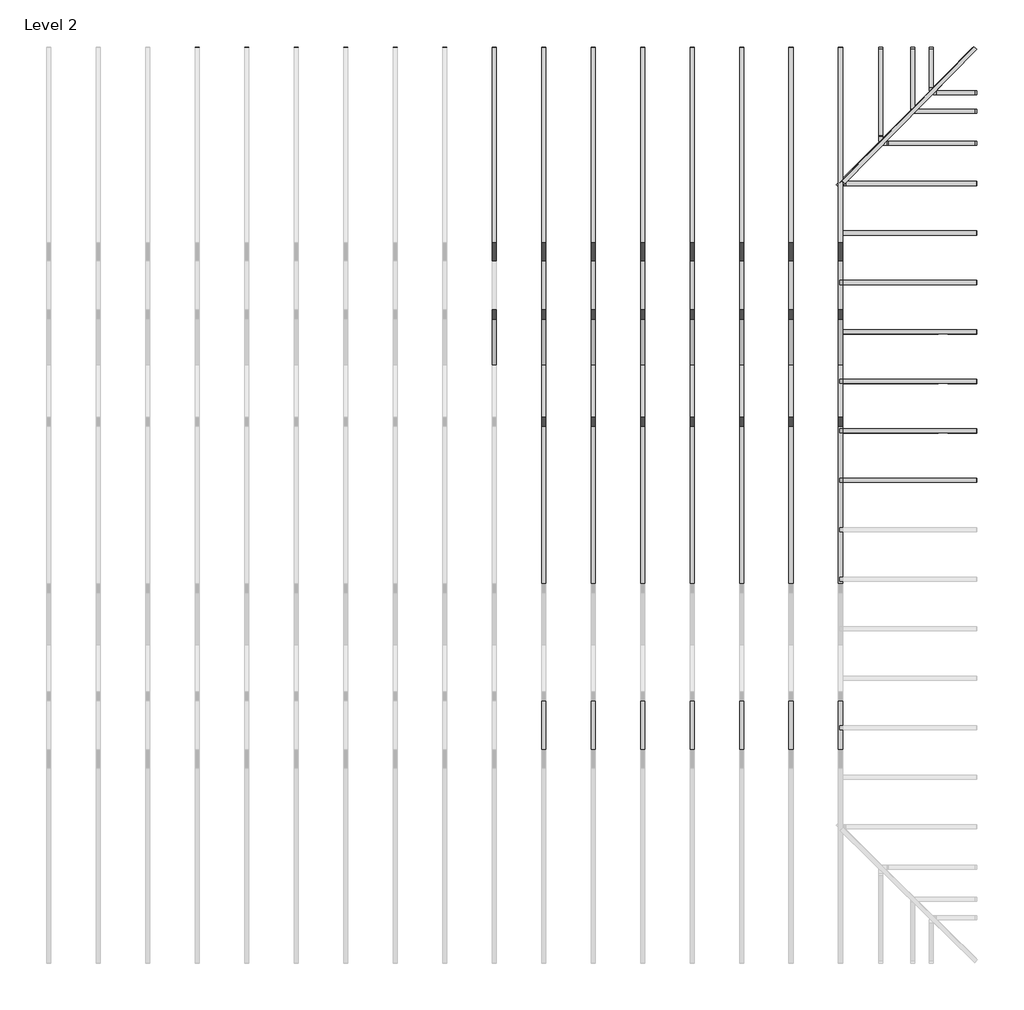
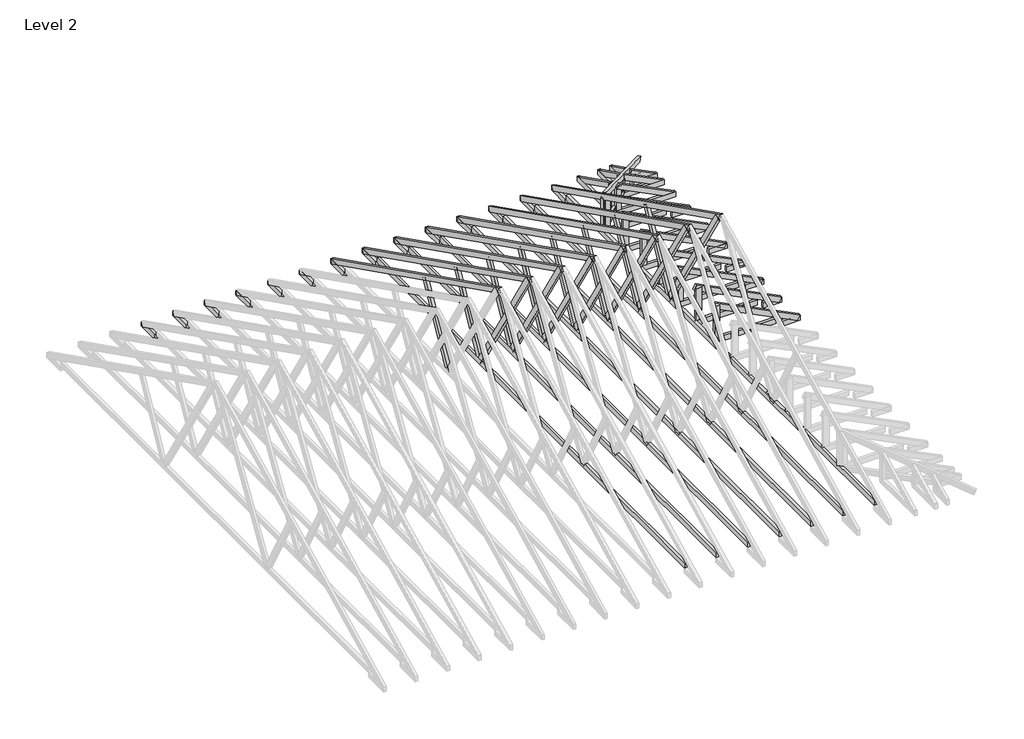
# One storey, part 5 of 5: 93 beams.
"""IFC4 building model written with IfcOpenShell, lengths in millimetres."""

import ifcopenshell
import ifcopenshell.guid

model = None  # the IFC model being written
_history = None  # IfcOwnerHistory: only IFC2X3 demands one
_inside = {}  # id of a spatial element -> (the spatial element, [elements in it])
_under = {}  # id of a project, library or spatial element -> (it, [spatial elements below it])
_declared = {}  # id of a project -> (the project, [libraries it declares])
_typed = {}  # id of a type object -> (the type object, [elements of that type])
_made_of = {}  # id of a material, layer set ... -> (it, [elements and type objects made of it])


def new_model(schema):
    """Start an empty IFC model of exactly this schema.

    Asked for "IFC4X3", IfcOpenShell would pick the latest addendum, in which some entities
    have other attributes; the version numbers below select the first issue.
    IFC2X3 requires an IfcOwnerHistory on every rooted entity: one is made here for all.
    """
    global model, _history
    if schema == "IFC4X3":
        model = ifcopenshell.file(schema_version=(4, 3, 0, 0))
    else:
        model = ifcopenshell.file(schema=schema)
    _inside.clear()
    _under.clear()
    _declared.clear()
    _typed.clear()
    _made_of.clear()
    _history = None
    if model.schema == "IFC2X3":
        org = make("IfcOrganization", Name="unknown")
        user = make(
            "IfcPersonAndOrganization",
            ThePerson=make("IfcPerson", FamilyName="unknown"),
            TheOrganization=org,
        )
        app = make(
            "IfcApplication",
            ApplicationDeveloper=org,
            Version="unknown",
            ApplicationFullName="unknown",
            ApplicationIdentifier="unknown",
        )
        _history = make(
            "IfcOwnerHistory",
            OwningUser=user,
            OwningApplication=app,
            ChangeAction="ADDED",
            CreationDate=0,
        )
    return model


def make(cls, **values):
    """One entity of the class cls with the attributes given. An attribute that is None is left unset."""
    return model.create_entity(
        cls, **{name: value for name, value in values.items() if value is not None}
    )


def rooted(cls, **values):
    """An entity with a GlobalId (a new one), such as an element, a storey or a relation."""
    return make(cls, GlobalId=ifcopenshell.guid.new(), OwnerHistory=_history, **values)


def si_unit(unit_type, name, prefix=None):
    """IfcSIUnit, for example si_unit("LENGTHUNIT", "METRE", prefix="MILLI")."""
    return make("IfcSIUnit", UnitType=unit_type, Prefix=prefix, Name=name)


def assignment(units):
    """IfcUnitAssignment: the units of a project."""
    return None if units is None else make("IfcUnitAssignment", Units=units)


def point(xyz):
    """IfcCartesianPoint."""
    return None if xyz is None else make("IfcCartesianPoint", Coordinates=xyz)


def direction(xyz):
    """IfcDirection."""
    return None if xyz is None else make("IfcDirection", DirectionRatios=xyz)


def frame(location, z_axis=None, x_axis=None):
    """IfcAxis2Placement3D, a coordinate frame: its origin and axes. An axis left out is left unset."""
    return make(
        "IfcAxis2Placement3D",
        Location=point(location),
        Axis=direction(z_axis),
        RefDirection=direction(x_axis),
    )


def origin():
    """The frame at (0, 0, 0) with its axes left unset."""
    return frame((0.0, 0.0, 0.0))


def place(relative_to, where):
    """IfcLocalPlacement: puts the frame where relative to a parent placement (None: the world)."""
    return make(
        "IfcLocalPlacement", PlacementRelTo=relative_to, RelativePlacement=where
    )


def context(
    kind, dimensions, precision=None, world=None, true_north=None, identifier=None
):
    """IfcGeometricRepresentationContext, for example the 3D "Model" context."""
    return make(
        "IfcGeometricRepresentationContext",
        ContextIdentifier=identifier,
        ContextType=kind,
        CoordinateSpaceDimension=dimensions,
        Precision=precision,
        WorldCoordinateSystem=world,
        TrueNorth=true_north,
    )


def project(units=None, contexts=None):
    """IfcProject with its units and contexts."""
    return rooted(
        "IfcProject",
        Name="project",
        RepresentationContexts=contexts,
        UnitsInContext=assignment(units),
    )


def spatial(cls, under=None, at=None, **own):
    """A site, building, storey or space (cls), placed at a placement, below another one or the project."""
    s = rooted(cls, ObjectPlacement=at, **own)
    if under is not None:
        _under.setdefault(under.id(), (under, []))[1].append(s)
    return s


def polyline(points):
    """IfcPolyline through the points."""
    return make("IfcPolyline", Points=[point(p) for p in points])


def outline(outer, holes=None, kind="AREA"):
    """IfcArbitraryClosedProfileDef: a profile drawn as a closed curve; with holes, ...WithVoids."""
    if holes is None:
        return make("IfcArbitraryClosedProfileDef", ProfileType=kind, OuterCurve=outer)
    return make(
        "IfcArbitraryProfileDefWithVoids",
        ProfileType=kind,
        OuterCurve=outer,
        InnerCurves=holes,
    )


def extrude(swept, where, along, depth):
    """IfcExtrudedAreaSolid: the profile swept, set in the frame where, extruded along a direction by depth."""
    return make(
        "IfcExtrudedAreaSolid",
        SweptArea=swept,
        Position=where,
        ExtrudedDirection=direction(along),
        Depth=depth,
    )


def shape(context_of_items, identifier, shape_type, items):
    """IfcShapeRepresentation: the items that make up one representation, for example the "Body"."""
    return make(
        "IfcShapeRepresentation",
        ContextOfItems=context_of_items,
        RepresentationIdentifier=identifier,
        RepresentationType=shape_type,
        Items=items,
    )


def source(mapping_origin, context_of_items, identifier, shape_type, items):
    """IfcRepresentationMap: a shape defined once, which mapped items show again and again."""
    return make(
        "IfcRepresentationMap",
        MappingOrigin=mapping_origin,
        MappedRepresentation=shape(context_of_items, identifier, shape_type, items),
    )


def transform(
    local_origin,
    x_axis=None,
    y_axis=None,
    z_axis=None,
    scale=None,
    scale2=None,
    scale3=None,
    uniform=True,
):
    """IfcCartesianTransformationOperator3D, or its non-uniform kind. x_axis, y_axis, z_axis: its Axis1, 2, 3."""
    if uniform:
        return make(
            "IfcCartesianTransformationOperator3D",
            Axis1=direction(x_axis),
            Axis2=direction(y_axis),
            LocalOrigin=point(local_origin),
            Scale=scale,
            Axis3=direction(z_axis),
        )
    return make(
        "IfcCartesianTransformationOperator3DnonUniform",
        Axis1=direction(x_axis),
        Axis2=direction(y_axis),
        LocalOrigin=point(local_origin),
        Scale=scale,
        Axis3=direction(z_axis),
        Scale2=scale2,
        Scale3=scale3,
    )


def mapped(mapping_source, mapping_target):
    """IfcMappedItem: shows the shape of a source again, moved by a transform."""
    return make(
        "IfcMappedItem", MappingSource=mapping_source, MappingTarget=mapping_target
    )


def made_of(thing, what):
    """Note that an element or type object is made of a material, layer set ...; save() writes the relation."""
    if what is not None:
        _made_of.setdefault(what.id(), (what, []))[1].append(thing)
    return thing


def element(
    cls,
    number,
    at=None,
    inside=None,
    cuts=None,
    type_object=None,
    material=None,
    context=None,
    identifier="Body",
    shape_type=None,
    held_by="IfcProductDefinitionShape",
    body=None,
    shapes=None,
    **own,
):
    """One element of the class cls, such as IfcWall. Its Tag is "e" and its number.

    at: its placement. inside: the storey or other place that contains it. cuts: it is an
    opening in that element (IfcRelVoidsElement). A single representation is given by context,
    identifier, shape_type and body (its items); several are given by shapes. held_by: the class
    of the entity that holds the representations. save() writes the other relations.
    """
    e = rooted(cls, Tag="e%d" % number, ObjectPlacement=at, **own)
    if body is not None:
        shapes = [shape(context, identifier, shape_type, body)]
    if shapes is not None:
        e.Representation = make(held_by, Representations=shapes)
    if inside is not None:
        _inside.setdefault(inside.id(), (inside, []))[1].append(e)
    if cuts is not None:
        rooted(
            "IfcRelVoidsElement", RelatingBuildingElement=cuts, RelatedOpeningElement=e
        )
    if type_object is not None:
        _typed.setdefault(type_object.id(), (type_object, []))[1].append(e)
    return made_of(e, material)


def aggregate(whole, parts):
    """IfcRelAggregates: a whole, such as a stair, and the parts it consists of."""
    return rooted("IfcRelAggregates", RelatingObject=whole, RelatedObjects=parts)


def save(model, path):
    """Write the relations noted so far, then the file.

    IfcRelAggregates (storeys below a building ...), IfcRelContainedInSpatialStructure (elements
    in a storey), IfcRelDefinesByType, IfcRelAssociatesMaterial and IfcRelDeclares: one each for
    every whole, place, type object, material and project.
    """
    for whole, parts in _under.values():
        aggregate(whole, parts)
    for where, things in _inside.values():
        rooted(
            "IfcRelContainedInSpatialStructure",
            RelatedElements=things,
            RelatingStructure=where,
        )
    for kind, things in _typed.values():
        rooted("IfcRelDefinesByType", RelatedObjects=things, RelatingType=kind)
    for what, things in _made_of.values():
        rooted("IfcRelAssociatesMaterial", RelatedObjects=things, RelatingMaterial=what)
    for by, libraries in _declared.values():
        rooted("IfcRelDeclares", RelatingContext=by, RelatedDefinitions=libraries)
    model.write(path)


def beam_b78a0881(model_context):
    return source(origin(), model_context, "Body", "SweptSolid", [
        extrude(outline(polyline([(228.6, 25.4), (228.6, -25.4), (-228.6, -25.4), (-228.6, 25.4), (228.6, 25.4)])), frame((0.0, 0.0, -50.8), z_axis=(0.0, 0.0, 1.0), x_axis=(1.0, 0.0, 0.0)), (0.0, 0.0, 1.0), 101.6),
    ])


def beam_85682148(model_context):
    return source(origin(), model_context, "Body", "SweptSolid", [
        extrude(outline(polyline([(595.8662636, -25.4), (-609.6, -25.4), (-609.6, 25.4), (595.8662636, 25.4), (595.8662636, -25.4)])), frame((0.0, 0.0, -50.8), z_axis=(0.0, 0.0, 1.0), x_axis=(1.0, 0.0, 0.0)), (0.0, 0.0, 1.0), 101.6),
    ])


def beam_f00f3f92(model_context):
    return source(origin(), model_context, "Body", "SweptSolid", [
        extrude(outline(polyline([(393.7, -25.4), (-393.7, -25.4), (-393.7, 25.4), (393.7, 25.4), (393.7, -25.4)])), frame((0.0, 0.0, -50.8), z_axis=(0.0, 0.0, 1.0), x_axis=(1.0, 0.0, 0.0)), (0.0, 0.0, 1.0), 101.6),
    ])


def beam_c3ddfe20(model_context):
    return source(origin(), model_context, "Body", "SweptSolid", [
        extrude(outline(polyline([(393.7, 25.4), (393.7, -25.4), (-368.3, -25.4), (-368.3, 25.4), (393.7, 25.4)])), frame((0.0, 0.0, -50.8), z_axis=(0.0, 0.0, 1.0), x_axis=(1.0, 0.0, 0.0)), (0.0, 0.0, 1.0), 101.6),
    ])


def beam_3de093d9(model_context):
    return source(origin(), model_context, "Body", "SweptSolid", [
        extrude(outline(polyline([(233.4866591, -25.4), (-1464.867127, -25.4), (-1464.867127, 25.4), (233.4866591, 25.4), (233.4866591, -25.4)])), frame((0.0, 0.0, -50.8), z_axis=(0.0, 0.0, 1.0), x_axis=(1.0, 0.0, 0.0)), (0.0, 0.0, 1.0), 101.6),
    ])


def beam_90eea034(model_context):
    return source(origin(), model_context, "Body", "SweptSolid", [
        extrude(outline(polyline([(821.193698, 25.4), (821.193698, -25.4), (-819.5010489, -25.4), (-819.5010489, 25.4), (821.193698, 25.4)])), frame((0.0, 0.0, -50.8), z_axis=(0.0, 0.0, 1.0), x_axis=(1.0, 0.0, 0.0)), (0.0, 0.0, 1.0), 101.6),
    ])


def beam_a4242642(model_context):
    return source(origin(), model_context, "Body", "SweptSolid", [
        extrude(outline(polyline([(5145.3336481, 25.4), (5145.3336481, -25.4), (-5145.3336481, -25.4), (-5145.3336481, 25.4), (5145.3336481, 25.4)])), frame((0.0, 0.0, -50.8), z_axis=(0.0, 0.0, 1.0), x_axis=(1.0, 0.0, 0.0)), (0.0, 0.0, 1.0), 101.6),
    ])


def beam_fc8bf4ae(model_context):
    return source(origin(), model_context, "Body", "SweptSolid", [
        extrude(outline(polyline([(1562.6646551, 25.4), (1562.6646551, -25.4), (-1550.1468127, -25.4), (-1550.1468127, 25.4), (1562.6646551, 25.4)])), frame((0.0, 0.0, -50.8), z_axis=(0.0, 0.0, 1.0), x_axis=(1.0, 0.0, 0.0)), (0.0, 0.0, 1.0), 101.6),
    ])


def beam_87710fdd(model_context):
    return source(origin(), model_context, "Body", "SweptSolid", [
        extrude(outline(polyline([(147.1272806, 25.4), (147.1272806, -25.4), (-142.875, -25.4), (-142.875, 25.4), (147.1272806, 25.4)])), frame((0.0, 0.0, -50.8), z_axis=(0.0, 0.0, 1.0), x_axis=(1.0, 0.0, 0.0)), (0.0, 0.0, 1.0), 101.6),
    ])


def beam_7b8fa6d1(model_context):
    return source(origin(), model_context, "Body", "SweptSolid", [
        extrude(outline(polyline([(270.7395597, 25.4), (270.7395597, -25.4), (-219.9395597, -25.4), (-219.9395597, 25.4), (270.7395597, 25.4)])), frame((0.0, 0.0, -50.8), z_axis=(0.0, 0.0, 1.0), x_axis=(1.0, 0.0, 0.0)), (0.0, 0.0, 1.0), 101.6),
    ])


def beam_42a29ae5(model_context):
    return source(origin(), model_context, "Body", "SweptSolid", [
        extrude(outline(polyline([(270.7395597, -25.4), (-219.9395597, -25.4), (-219.9395597, 25.4), (270.7395597, 25.4), (270.7395597, -25.4)])), frame((0.0, 0.0, -50.8), z_axis=(0.0, 0.0, 1.0), x_axis=(1.0, 0.0, 0.0)), (0.0, 0.0, 1.0), 101.6),
    ])


def beam_11c5b8ca(model_context):
    return source(origin(), model_context, "Body", "SweptSolid", [
        extrude(outline(polyline([(147.1272806, -25.4), (-142.875, -25.4), (-142.875, 25.4), (147.1272806, 25.4), (147.1272806, -25.4)])), frame((0.0, 0.0, -50.8), z_axis=(0.0, 0.0, 1.0), x_axis=(1.0, 0.0, 0.0)), (0.0, 0.0, 1.0), 101.6),
    ])


def beam_a8bd1fc0(model_context):
    return source(origin(), model_context, "Body", "SweptSolid", [
        extrude(outline(polyline([(571.5, -25.4), (-609.6, -25.4), (-609.6, 25.4), (571.5, 25.4), (571.5, -25.4)])), frame((0.0, 0.0, -50.8), z_axis=(0.0, 0.0, 1.0), x_axis=(1.0, 0.0, 0.0)), (0.0, 0.0, 1.0), 101.6),
    ])


def beam_f5027b49(model_context):
    return source(origin(), model_context, "Body", "SweptSolid", [
        extrude(outline(polyline([(571.5, 25.4), (571.5, -25.4), (-584.2, -25.4), (-584.2, 25.4), (571.5, 25.4)])), frame((0.0, 0.0, -50.8), z_axis=(0.0, 0.0, 1.0), x_axis=(1.0, 0.0, 0.0)), (0.0, 0.0, 1.0), 101.6),
    ])


def beam_78ff79ac(model_context):
    return source(origin(), model_context, "Body", "SweptSolid", [
        extrude(outline(polyline([(365.3019367, -25.4), (-314.5019367, -25.4), (-314.5019367, 25.4), (365.3019367, 25.4), (365.3019367, -25.4)])), frame((0.0, 0.0, -50.8), z_axis=(0.0, 0.0, 1.0), x_axis=(1.0, 0.0, 0.0)), (0.0, 0.0, 1.0), 101.6),
    ])


def beam_99e5442a(model_context):
    return source(origin(), model_context, "Body", "SweptSolid", [
        extrude(outline(polyline([(350.5042173, -25.4), (-295.4519367, -25.4), (-295.4519367, 25.4), (350.5042173, 25.4), (350.5042173, -25.4)])), frame((0.0, 0.0, -50.8), z_axis=(0.0, 0.0, 1.0), x_axis=(1.0, 0.0, 0.0)), (0.0, 0.0, 1.0), 101.6),
    ])


def beam_38e3f9e5(model_context):
    return source(origin(), model_context, "Body", "SweptSolid", [
        extrude(outline(polyline([(595.8662636, -25.4), (-548.2789755, -25.4), (-548.2789755, 25.4), (595.8662636, 25.4), (595.8662636, -25.4)])), frame((0.0, 0.0, -50.8), z_axis=(0.0, 0.0, 1.0), x_axis=(1.0, 0.0, 0.0)), (0.0, 0.0, 1.0), 101.6),
    ])


def beam_7aad778a(model_context):
    return source(origin(), model_context, "Body", "SweptSolid", [
        extrude(outline(polyline([(307.975, -25.4), (-47.625, -25.4), (-47.625, 25.4), (307.975, 25.4), (307.975, -25.4)])), frame((0.0, 0.0, -50.8), z_axis=(0.0, 0.0, 1.0), x_axis=(1.0, 0.0, 0.0)), (0.0, 0.0, 1.0), 101.6),
    ])


def beam_878446a4(model_context):
    return source(origin(), model_context, "Body", "SweptSolid", [
        extrude(outline(polyline([(63.8057136, 25.4), (63.8057136, -25.4), (-59.553433, -25.4), (-59.553433, 25.4), (63.8057136, 25.4)])), frame((0.0, 0.0, -50.8), z_axis=(0.0, 0.0, 1.0), x_axis=(1.0, 0.0, 0.0)), (0.0, 0.0, 1.0), 101.6),
    ])


def beam_bc99fd75(model_context):
    return source(origin(), model_context, "Body", "SweptSolid", [
        extrude(outline(polyline([(222.3387319, 25.4), (222.3387319, -25.4), (-231.775, -25.4), (-231.775, 25.4), (222.3387319, 25.4)])), frame((0.0, 0.0, -50.8), z_axis=(0.0, 0.0, 1.0), x_axis=(1.0, 0.0, 0.0)), (0.0, 0.0, 1.0), 101.6),
    ])


def beam_efe25585(model_context):
    return source(origin(), model_context, "Body", "SweptSolid", [
        extrude(outline(polyline([(222.3387319, -25.4), (-231.775, -25.4), (-231.775, 25.4), (222.3387319, 25.4), (222.3387319, -25.4)])), frame((0.0, 0.0, -50.8), z_axis=(0.0, 0.0, 1.0), x_axis=(1.0, 0.0, 0.0)), (0.0, 0.0, 1.0), 101.6),
    ])


def beam_dfed05dc(model_context):
    return source(origin(), model_context, "Body", "SweptSolid", [
        extrude(outline(polyline([(63.8057136, -25.4), (-59.553433, -25.4), (-59.553433, 25.4), (63.8057136, 25.4), (63.8057136, -25.4)])), frame((0.0, 0.0, -50.8), z_axis=(0.0, 0.0, 1.0), x_axis=(1.0, 0.0, 0.0)), (0.0, 0.0, 1.0), 101.6),
    ])


model = new_model("IFC4")

# Units and contexts
model_context = context("Model", 3, world=origin())
ifc_project = project(units=[si_unit("LENGTHUNIT", "METRE", prefix="MILLI")], contexts=[model_context])

# Site, building, storey
site = spatial("IfcSite", under=ifc_project)
building = spatial("IfcBuilding", under=site)
storey = spatial("IfcBuildingStorey", under=building, Name="Level 2", Elevation=2768.6)

# Beams
placement = place(None, origin())
element("IfcBeam", 1, ObjectType="Dimension Lumber : BLDG 6241 2X4\" TRUSS MEMBER", at=placement, inside=storey, context=model_context, shape_type="SweptSolid", body=[
    extrude(outline(polyline([(0.0, -50.8), (0.0, 0.0), (6302.2496334, 0.0), (6302.2496334, -50.8), (0.0, -50.8)])), frame((-3805.814829, -17.2791662, 5496.1115355), z_axis=(0.0, 0.4472135954999557, 0.894427190999917), x_axis=(0.0, 0.894427190999917, -0.4472135954999557)), (0.0, 0.0, 1.0), 101.6),
])
element("IfcBeam", 2, ObjectType="Dimension Lumber : BLDG 6241 2X4\" TRUSS MEMBER", at=placement, inside=storey, context=model_context, shape_type="SweptSolid", body=[
    extrude(outline(polyline([(0.0, -50.8), (0.0, 0.0), (6302.2496334, 0.0), (6302.2496334, -50.8), (0.0, -50.8)])), frame((-3196.214829, -17.2791662, 5496.1115355), z_axis=(0.0, 0.4472135954999561, 0.8944271909999169), x_axis=(0.0, 0.8944271909999169, -0.4472135954999561)), (0.0, 0.0, 1.0), 101.6),
])
element("IfcBeam", 3, ObjectType="Dimension Lumber : BLDG 6241 2X4\" TRUSS MEMBER", at=placement, inside=storey, context=model_context, shape_type="SweptSolid", body=[
    extrude(outline(polyline([(0.0, -50.8), (0.0, 0.0), (6302.2496334, 0.0), (6302.2496334, -50.8), (0.0, -50.8)])), frame((-2586.614829, -17.2791662, 5496.1115355), z_axis=(0.0, 0.44721359549995593, 0.894427190999917), x_axis=(0.0, 0.894427190999917, -0.44721359549995593)), (0.0, 0.0, 1.0), 101.6),
])
element("IfcBeam", 4, ObjectType="Dimension Lumber : BLDG 6241 2X4\" TRUSS MEMBER", at=placement, inside=storey, context=model_context, shape_type="SweptSolid", body=[
    extrude(outline(polyline([(0.0, -50.8), (0.0, 0.0), (6302.2496334, 0.0), (6302.2496334, -50.8), (0.0, -50.8)])), frame((-1977.014829, -17.2791662, 5496.1115355), z_axis=(0.0, 0.447213595499956, 0.8944271909999169), x_axis=(0.0, 0.8944271909999169, -0.447213595499956)), (0.0, 0.0, 1.0), 101.6),
])
element("IfcBeam", 5, ObjectType="Dimension Lumber : BLDG 6241 2X4\" TRUSS MEMBER", at=placement, inside=storey, context=model_context, shape_type="SweptSolid", body=[
    extrude(outline(polyline([(0.0, -50.8), (0.0, 0.0), (6302.2496334, 0.0), (6302.2496334, -50.8), (0.0, -50.8)])), frame((-1367.414829, -17.2791662, 5496.1115355), z_axis=(0.0, 0.44721359549995593, 0.894427190999917), x_axis=(0.0, 0.894427190999917, -0.44721359549995593)), (0.0, 0.0, 1.0), 101.6),
])
element("IfcBeam", 6, ObjectType="Dimension Lumber : BLDG 6241 2X4\" TRUSS MEMBER", at=placement, inside=storey, context=model_context, shape_type="SweptSolid", body=[
    extrude(outline(polyline([(0.0, -50.8), (0.0, 0.0), (6302.2496334, 0.0), (6302.2496334, -50.8), (0.0, -50.8)])), frame((-757.814829, -17.2791662, 5496.1115355), z_axis=(0.0, 0.4472135954999558, 0.894427190999917), x_axis=(0.0, 0.894427190999917, -0.4472135954999558)), (0.0, 0.0, 1.0), 101.6),
])
element("IfcBeam", 7, ObjectType="Dimension Lumber : BLDG 6241 2X4\" TRUSS MEMBER", at=placement, inside=storey, context=model_context, shape_type="SweptSolid", body=[
    extrude(outline(polyline([(0.0, -50.8), (0.0, 0.0), (6302.2496334, 0.0), (6302.2496334, -50.8), (0.0, -50.8)])), frame((-148.214829, -17.2791662, 5496.1115355), z_axis=(0.0, 0.4472135954999557, 0.894427190999917), x_axis=(0.0, 0.894427190999917, -0.4472135954999557)), (0.0, 0.0, 1.0), 101.6),
])
element("IfcBeam", 8, ObjectType="Dimension Lumber : BLDG 6241 2X4\" TRUSS MEMBER", at=placement, inside=storey, context=model_context, shape_type="SweptSolid", body=[
    extrude(outline(polyline([(0.0, -50.8), (0.0, 0.0), (6302.2496334, 0.0), (6302.2496334, -50.8), (0.0, -50.8)])), frame((461.385171, -17.2791662, 5496.1115355), z_axis=(0.0, 0.4472135954999561, 0.8944271909999169), x_axis=(0.0, 0.8944271909999169, -0.4472135954999561)), (0.0, 0.0, 1.0), 101.6),
])
element("IfcBeam", 9, ObjectType="Dimension Lumber : BLDG 6241 2X4\" TRUSS MEMBER", at=placement, inside=storey, context=model_context, shape_type="SweptSolid", body=[
    extrude(outline(polyline([(0.0, 50.8), (1828.8, 50.8), (1828.8, 0.0), (0.0, 0.0), (0.0, 50.8)])), frame((2110.9853106, 3404.3284114, 2681.1076769), z_axis=(0.44721359549995937, 0.0, 0.8944271909999152), x_axis=(-0.8944271909999152, 0.0, 0.44721359549995937)), (0.0, 0.0, 1.0), 101.6),
])
element("IfcBeam", 10, ObjectType="Dimension Lumber : BLDG 6241 2X4\" TRUSS MEMBER", at=placement, inside=storey, context=model_context, shape_type="SweptSolid", body=[
    extrude(outline(polyline([(0.0, 50.8000001), (2461.5286969, 50.8), (2461.528697, 0.0), (0.0, 0.0), (0.0, 50.8000001)])), frame((510.3258967, 3962.9132559, 3515.7397288), z_axis=(0.25320527715849206, 0.22183093198504344, 0.9416358772018716), x_axis=(0.6604274920267093, 0.6716162760239278, -0.33580813801196396)), (0.0, 0.0, 1.0), 101.6),
])
element("IfcBeam", 11, ObjectType="Dimension Lumber : BLDG 6241 2X4\" TRUSS MEMBER", at=placement, inside=storey, context=model_context, shape_type="SweptSolid", body=[
    extrude(outline(polyline([(0.0, 50.8), (1203.6219076, 50.8), (1203.6219076, 0.0), (0.0, 0.0), (0.0, 50.8)])), frame((2112.5153243, 4509.2284114, 2680.3426701), z_axis=(0.44721359549995937, 0.0, 0.8944271909999152), x_axis=(-0.8944271909999152, 0.0, 0.44721359549995937)), (0.0, 0.0, 1.0), 101.6),
])
element("IfcBeam", 12, ObjectType="Dimension Lumber : BLDG 6241 2X4\" TRUSS MEMBER", at=placement, inside=storey, context=model_context, shape_type="SweptSolid", body=[
    extrude(outline(polyline([(0.0, 50.8), (844.55, 50.8), (844.55, 0.0), (0.0, 0.0), (0.0, 50.8)])), frame((2117.2589031, 4902.9284114, 2677.9708807), z_axis=(0.4472135954999599, 0.0, 0.894427190999915), x_axis=(-0.894427190999915, 0.0, 0.4472135954999599)), (0.0, 0.0, 1.0), 101.6),
])
element("IfcBeam", 13, ObjectType="Dimension Lumber : BLDG 6241 2X4\" TRUSS MEMBER", at=placement, inside=storey, context=model_context, shape_type="SweptSolid", body=[
    extrude(outline(polyline([(0.0, 50.8), (1787.5128973, 50.8), (1787.5128973, 0.0), (0.0, 0.0), (0.0, 50.8)])), frame((2110.9853106, 4013.9284114, 2681.1076769), z_axis=(0.44721359549995937, 0.0, 0.8944271909999152), x_axis=(-0.8944271909999152, 0.0, 0.44721359549995937)), (0.0, 0.0, 1.0), 101.6),
])
element("IfcBeam", 14, ObjectType="Dimension Lumber : BLDG 6241 2X4\" TRUSS MEMBER", at=placement, inside=storey, context=model_context, shape_type="SweptSolid", body=[
    extrude(outline(polyline([(0.0, 50.8), (1828.8, 50.8), (1828.8, 0.0), (0.0, 0.0), (0.0, 50.8)])), frame((2110.9853106, 2794.7284114, 2681.1076769), z_axis=(0.44721359549995937, 0.0, 0.8944271909999152), x_axis=(-0.8944271909999152, 0.0, 0.44721359549995937)), (0.0, 0.0, 1.0), 101.6),
])
element("IfcBeam", 15, ObjectType="Dimension Lumber : BLDG 6241 2X4\" TRUSS MEMBER", at=placement, inside=storey, context=model_context, shape_type="SweptSolid", body=[
    extrude(outline(polyline([(0.0, 50.8), (1828.8, 50.8), (1828.8, 0.0), (0.0, 0.0), (0.0, 50.8)])), frame((2110.9853106, 2185.1284114, 2681.1076769), z_axis=(0.44721359549995937, 0.0, 0.8944271909999152), x_axis=(-0.8944271909999152, 0.0, 0.44721359549995937)), (0.0, 0.0, 1.0), 101.6),
])
element("IfcBeam", 16, ObjectType="Dimension Lumber : BLDG 6241 2X4\" TRUSS MEMBER", at=placement, inside=storey, context=model_context, shape_type="SweptSolid", body=[
    extrude(outline(polyline([(0.0, 50.8), (1828.8, 50.8), (1828.8, 0.0), (0.0, 0.0), (0.0, 50.8)])), frame((2110.9853106, 1575.5284114, 2681.1076769), z_axis=(0.44721359549995937, 0.0, 0.8944271909999152), x_axis=(-0.8944271909999152, 0.0, 0.44721359549995937)), (0.0, 0.0, 1.0), 101.6),
])
element("IfcBeam", 17, ObjectType="Dimension Lumber : BLDG 6241 2X4\" TRUSS MEMBER", at=placement, inside=storey, context=model_context, shape_type="SweptSolid", body=[
    extrude(outline(polyline([(0.0, 50.8), (1828.8, 50.8), (1828.8, 0.0), (0.0, 0.0), (0.0, 50.8)])), frame((2110.9853106, 965.9284114, 2681.1076769), z_axis=(0.44721359549995937, 0.0, 0.8944271909999152), x_axis=(-0.8944271909999152, 0.0, 0.44721359549995937)), (0.0, 0.0, 1.0), 101.6),
])
element("IfcBeam", 18, ObjectType="Dimension Lumber : BLDG 6241 2X4\" TRUSS MEMBER", at=placement, inside=storey, context=model_context, shape_type="SweptSolid", body=[
    extrude(outline(polyline([(0.0, 50.8), (1828.8, 50.8), (1828.8, 0.0), (0.0, 0.0), (0.0, 50.8)])), frame((2110.9853106, 356.3284114, 2681.1076769), z_axis=(0.44721359549995937, 0.0, 0.8944271909999152), x_axis=(-0.8944271909999152, 0.0, 0.44721359549995937)), (0.0, 0.0, 1.0), 101.6),
])
element("IfcBeam", 19, ObjectType="Dimension Lumber : BLDG 6241 2X4\" TRUSS MEMBER", at=placement, inside=storey, context=model_context, shape_type="SweptSolid", body=[
    extrude(outline(polyline([(0.0, -50.8), (0.0, 0.0), (1203.6219076, 0.0), (1203.6219076, -50.8), (0.0, -50.8)])), frame((1007.485171, 5614.2585647, 2680.3426701), z_axis=(0.0, 0.44721359549995937, 0.8944271909999152), x_axis=(0.0, -0.8944271909999152, 0.44721359549995937)), (0.0, 0.0, 1.0), 101.6),
])
element("IfcBeam", 20, ObjectType="Dimension Lumber : BLDG 6241 2X4\" TRUSS MEMBER", at=placement, inside=storey, context=model_context, shape_type="SweptSolid", body=[
    extrude(outline(polyline([(0.0, -50.8), (0.0, 0.0), (844.55, 0.0), (844.55, -50.8), (0.0, -50.8)])), frame((1401.185171, 5619.0021435, 2677.9708807), z_axis=(0.0, 0.4472135954999599, 0.894427190999915), x_axis=(0.0, -0.894427190999915, 0.4472135954999599)), (0.0, 0.0, 1.0), 101.6),
])
element("IfcBeam", 21, ObjectType="Dimension Lumber : BLDG 6241 2X4\" TRUSS MEMBER", at=placement, inside=storey, context=model_context, shape_type="SweptSolid", body=[
    extrude(outline(polyline([(0.0, 50.8), (546.1, 50.8), (546.1, 0.0), (0.0, 0.0), (0.0, 50.8)])), frame((2116.9461224, 5131.5284114, 2678.127271), z_axis=(0.4472135954999593, 0.0, 0.8944271909999153), x_axis=(-0.8944271909999153, 0.0, 0.4472135954999593)), (0.0, 0.0, 1.0), 101.6),
])
element("IfcBeam", 22, ObjectType="Dimension Lumber : BLDG 6241 2X4\" TRUSS MEMBER", at=placement, inside=storey, context=model_context, shape_type="SweptSolid", body=[
    extrude(outline(polyline([(0.0, -50.8), (0.0, 0.0), (546.1, 0.0), (546.1, -50.8), (0.0, -50.8)])), frame((1629.785171, 5618.6893628, 2678.127271), z_axis=(0.0, 0.4472135954999592, 0.8944271909999153), x_axis=(0.0, -0.8944271909999153, 0.4472135954999592)), (0.0, 0.0, 1.0), 101.6),
])
beam_shape = beam_b78a0881(model_context)
element("IfcBeam", 23, ObjectType="Dimension Lumber : BLDG 6241 2X4\" TRUSS MEMBER", at=placement, inside=storey, context=model_context, shape_type="MappedRepresentation", body=[
    mapped(beam_shape, transform((-7438.014829, 5436.3284114, 2717.8), x_axis=(0.0, -1.0, 0.0), y_axis=(1.0, 0.0, 0.0), z_axis=(0.0, 0.0, 1.0))),
])
element("IfcBeam", 24, ObjectType="Dimension Lumber : BLDG 6241 2X4\" TRUSS MEMBER", at=placement, inside=storey, context=model_context, shape_type="MappedRepresentation", body=[
    mapped(beam_shape, transform((-6828.414829, 5436.3284114, 2717.8), x_axis=(0.0, -1.0, 0.0), y_axis=(1.0, 0.0, 0.0), z_axis=(0.0, 0.0, 1.0))),
])
element("IfcBeam", 25, ObjectType="Dimension Lumber : BLDG 6241 2X4\" TRUSS MEMBER", at=placement, inside=storey, context=model_context, shape_type="MappedRepresentation", body=[
    mapped(beam_shape, transform((-6218.814829, 5436.3284114, 2717.8), x_axis=(0.0, -1.0, 0.0), y_axis=(1.0, 0.0, 0.0), z_axis=(0.0, 0.0, 1.0))),
])
element("IfcBeam", 26, ObjectType="Dimension Lumber : BLDG 6241 2X4\" TRUSS MEMBER", at=placement, inside=storey, context=model_context, shape_type="MappedRepresentation", body=[
    mapped(beam_shape, transform((-5609.214829, 5436.3284114, 2717.8), x_axis=(0.0, -1.0, 0.0), y_axis=(1.0, 0.0, 0.0), z_axis=(0.0, 0.0, 1.0))),
])
element("IfcBeam", 27, ObjectType="Dimension Lumber : BLDG 6241 2X4\" TRUSS MEMBER", at=placement, inside=storey, context=model_context, shape_type="MappedRepresentation", body=[
    mapped(beam_shape, transform((-4999.614829, 5436.3284114, 2717.8), x_axis=(0.0, -1.0, 0.0), y_axis=(1.0, 0.0, 0.0), z_axis=(0.0, 0.0, 1.0))),
])
element("IfcBeam", 28, ObjectType="Dimension Lumber : BLDG 6241 2X4\" TRUSS MEMBER", at=placement, inside=storey, context=model_context, shape_type="MappedRepresentation", body=[
    mapped(beam_shape, transform((-4390.014829, 5436.3284114, 2717.8), x_axis=(0.0, -1.0, 0.0), y_axis=(1.0, 0.0, 0.0), z_axis=(0.0, 0.0, 1.0))),
])
element("IfcBeam", 29, ObjectType="Dimension Lumber : BLDG 6241 2X4\" TRUSS MEMBER", at=placement, inside=storey, context=model_context, shape_type="MappedRepresentation", body=[
    mapped(beam_shape, transform((-3780.414829, 5436.3284114, 2717.8), x_axis=(0.0, -1.0, 0.0), y_axis=(1.0, 0.0, 0.0), z_axis=(0.0, 0.0, 1.0))),
])
element("IfcBeam", 30, ObjectType="Dimension Lumber : BLDG 6241 2X4\" TRUSS MEMBER", at=placement, inside=storey, context=model_context, shape_type="MappedRepresentation", body=[
    mapped(beam_shape, transform((-3170.814829, 5436.3284114, 2717.8), x_axis=(0.0, -1.0, 0.0), y_axis=(1.0, 0.0, 0.0), z_axis=(0.0, 0.0, 1.0))),
])
element("IfcBeam", 31, ObjectType="Dimension Lumber : BLDG 6241 2X4\" TRUSS MEMBER", at=placement, inside=storey, context=model_context, shape_type="MappedRepresentation", body=[
    mapped(beam_shape, transform((-2561.214829, 5436.3284114, 2717.8), x_axis=(0.0, -1.0, 0.0), y_axis=(1.0, 0.0, 0.0), z_axis=(0.0, 0.0, 1.0))),
])
element("IfcBeam", 32, ObjectType="Dimension Lumber : BLDG 6241 2X4\" TRUSS MEMBER", at=placement, inside=storey, context=model_context, shape_type="MappedRepresentation", body=[
    mapped(beam_shape, transform((-1951.614829, 5436.3284114, 2717.8), x_axis=(0.0, -1.0, 0.0), y_axis=(1.0, 0.0, 0.0), z_axis=(0.0, 0.0, 1.0))),
])
element("IfcBeam", 33, ObjectType="Dimension Lumber : BLDG 6241 2X4\" TRUSS MEMBER", at=placement, inside=storey, context=model_context, shape_type="MappedRepresentation", body=[
    mapped(beam_shape, transform((-1342.014829, 5436.3284114, 2717.8), x_axis=(0.0, -1.0, 0.0), y_axis=(1.0, 0.0, 0.0), z_axis=(0.0, 0.0, 1.0))),
])
element("IfcBeam", 34, ObjectType="Dimension Lumber : BLDG 6241 2X4\" TRUSS MEMBER", at=placement, inside=storey, context=model_context, shape_type="MappedRepresentation", body=[
    mapped(beam_shape, transform((-732.414829, 5436.3284114, 2717.8), x_axis=(0.0, -1.0, 0.0), y_axis=(1.0, 0.0, 0.0), z_axis=(0.0, 0.0, 1.0))),
])
element("IfcBeam", 35, ObjectType="Dimension Lumber : BLDG 6241 2X4\" TRUSS MEMBER", at=placement, inside=storey, context=model_context, shape_type="MappedRepresentation", body=[
    mapped(beam_shape, transform((-122.814829, 5436.3284114, 2717.8), x_axis=(0.0, -1.0, 0.0), y_axis=(1.0, 0.0, 0.0), z_axis=(0.0, 0.0, 1.0))),
])
element("IfcBeam", 36, ObjectType="Dimension Lumber : BLDG 6241 2X4\" TRUSS MEMBER", at=placement, inside=storey, context=model_context, shape_type="MappedRepresentation", body=[
    mapped(beam_shape, transform((486.785171, 5436.3284114, 2717.8), x_axis=(0.0, -1.0, 0.0), y_axis=(1.0, 0.0, 0.0), z_axis=(0.0, 0.0, 1.0))),
])
beam_2_shape = beam_85682148(model_context)
element("IfcBeam", 37, ObjectType="Dimension Lumber : BLDG 6241 2X4\" TRUSS MEMBER", at=placement, inside=storey, context=model_context, shape_type="MappedRepresentation", body=[
    mapped(beam_2_shape, transform((1096.385171, 3378.9284114, 2819.4), x_axis=(1.0, 0.0, 0.0), y_axis=(0.0, 1.0, 0.0), z_axis=(0.0, 0.0, 1.0))),
])
element("IfcBeam", 38, ObjectType="Dimension Lumber : BLDG 6241 2X4\" TRUSS MEMBER", at=placement, inside=storey, context=model_context, shape_type="MappedRepresentation", body=[
    mapped(beam_2_shape, transform((1096.385171, 2769.3284114, 2819.4), x_axis=(1.0, 0.0, 0.0), y_axis=(0.0, 1.0, 0.0), z_axis=(0.0, 0.0, 1.0))),
])
element("IfcBeam", 39, ObjectType="Dimension Lumber : BLDG 6241 2X4\" TRUSS MEMBER", at=placement, inside=storey, context=model_context, shape_type="MappedRepresentation", body=[
    mapped(beam_2_shape, transform((1096.385171, 2159.7284114, 2819.4), x_axis=(1.0, 0.0, 0.0), y_axis=(0.0, 1.0, 0.0), z_axis=(0.0, 0.0, 1.0))),
])
element("IfcBeam", 40, ObjectType="Dimension Lumber : BLDG 6241 2X4\" TRUSS MEMBER", at=placement, inside=storey, context=model_context, shape_type="MappedRepresentation", body=[
    mapped(beam_2_shape, transform((1096.385171, 1550.1284114, 2819.4), x_axis=(1.0, 0.0, 0.0), y_axis=(0.0, 1.0, 0.0), z_axis=(0.0, 0.0, 1.0))),
])
element("IfcBeam", 41, ObjectType="Dimension Lumber : BLDG 6241 2X4\" TRUSS MEMBER", at=placement, inside=storey, context=model_context, shape_type="MappedRepresentation", body=[
    mapped(beam_2_shape, transform((1096.385171, 940.5284114, 2819.4), x_axis=(1.0, 0.0, 0.0), y_axis=(0.0, 1.0, 0.0), z_axis=(0.0, 0.0, 1.0))),
])
element("IfcBeam", 42, ObjectType="Dimension Lumber : BLDG 6241 2X4\" TRUSS MEMBER", at=placement, inside=storey, context=model_context, shape_type="MappedRepresentation", body=[
    mapped(beam_2_shape, transform((1096.385171, 330.9284114, 2819.4), x_axis=(1.0, 0.0, 0.0), y_axis=(0.0, 1.0, 0.0), z_axis=(0.0, 0.0, 1.0))),
])
beam_3_shape = beam_f00f3f92(model_context)
element("IfcBeam", 43, ObjectType="Dimension Lumber : BLDG 6241 2X4\" TRUSS MEMBER", at=placement, inside=storey, context=model_context, shape_type="MappedRepresentation", body=[
    mapped(beam_3_shape, transform((1769.485171, 4877.5284114, 2728.7708807), x_axis=(1.0, 0.0, 0.0), y_axis=(0.0, 1.0, 0.0), z_axis=(0.0, 0.0, 1.0))),
])
beam_4_shape = beam_c3ddfe20(model_context)
element("IfcBeam", 44, ObjectType="Dimension Lumber : BLDG 6241 2X4\" TRUSS MEMBER", at=placement, inside=storey, context=model_context, shape_type="MappedRepresentation", body=[
    mapped(beam_4_shape, transform((1375.785171, 5271.2284114, 2728.7708807), x_axis=(0.0, 1.0, 0.0), y_axis=(-1.0, 0.0, 0.0), z_axis=(0.0, 0.0, 1.0))),
])
beam_5_shape = beam_3de093d9(model_context)
element("IfcBeam", 45, ObjectType="Dimension Lumber : BLDG 6241 2X4\" TRUSS MEMBER", at=placement, inside=storey, context=model_context, shape_type="MappedRepresentation", body=[
    mapped(beam_5_shape, transform((677.285171, 4179.0284114, 2819.4), x_axis=(-0.7071067811865462, -0.7071067811865488, 0.0), y_axis=(0.7071067811865488, -0.7071067811865462, 0.0), z_axis=(0.0, 0.0, 1.0))),
])
beam_6_shape = beam_90eea034(model_context)
element("IfcBeam", 46, ObjectType="Dimension Lumber : BLDG 6241 2X4\" TRUSS MEMBER", at=placement, inside=storey, context=model_context, shape_type="MappedRepresentation", body=[
    mapped(beam_6_shape, transform((-3780.414829, 2147.8781861, 3552.5770493), x_axis=(0.0, -0.4803172630852004, -0.8770948220017847), y_axis=(-1.0, 0.0, 0.0), z_axis=(0.0, 0.8770948220017847, -0.4803172630852004))),
])
element("IfcBeam", 47, ObjectType="Dimension Lumber : BLDG 6241 2X4\" TRUSS MEMBER", at=placement, inside=storey, context=model_context, shape_type="MappedRepresentation", body=[
    mapped(beam_6_shape, transform((-3170.814829, 2147.8781861, 3552.5770493), x_axis=(0.0, -0.4803172630852004, -0.8770948220017847), y_axis=(-1.0, 0.0, 0.0), z_axis=(0.0, 0.8770948220017847, -0.4803172630852004))),
])
element("IfcBeam", 48, ObjectType="Dimension Lumber : BLDG 6241 2X4\" TRUSS MEMBER", at=placement, inside=storey, context=model_context, shape_type="MappedRepresentation", body=[
    mapped(beam_6_shape, transform((-2561.214829, 2147.8781861, 3552.5770493), x_axis=(0.0, -0.4803172630852004, -0.8770948220017847), y_axis=(-1.0, 0.0, 0.0), z_axis=(0.0, 0.8770948220017847, -0.4803172630852004))),
])
element("IfcBeam", 49, ObjectType="Dimension Lumber : BLDG 6241 2X4\" TRUSS MEMBER", at=placement, inside=storey, context=model_context, shape_type="MappedRepresentation", body=[
    mapped(beam_6_shape, transform((-1951.614829, 2147.8781861, 3552.5770493), x_axis=(0.0, -0.4803172630852004, -0.8770948220017847), y_axis=(-1.0, 0.0, 0.0), z_axis=(0.0, 0.8770948220017847, -0.4803172630852004))),
])
element("IfcBeam", 50, ObjectType="Dimension Lumber : BLDG 6241 2X4\" TRUSS MEMBER", at=placement, inside=storey, context=model_context, shape_type="MappedRepresentation", body=[
    mapped(beam_6_shape, transform((-1342.014829, 2147.8781861, 3552.5770493), x_axis=(0.0, -0.4803172630852004, -0.8770948220017847), y_axis=(-1.0, 0.0, 0.0), z_axis=(0.0, 0.8770948220017847, -0.4803172630852004))),
])
element("IfcBeam", 51, ObjectType="Dimension Lumber : BLDG 6241 2X4\" TRUSS MEMBER", at=placement, inside=storey, context=model_context, shape_type="MappedRepresentation", body=[
    mapped(beam_6_shape, transform((-732.414829, 2147.8781861, 3552.5770493), x_axis=(0.0, -0.4803172630852004, -0.8770948220017847), y_axis=(-1.0, 0.0, 0.0), z_axis=(0.0, 0.8770948220017847, -0.4803172630852004))),
])
element("IfcBeam", 52, ObjectType="Dimension Lumber : BLDG 6241 2X4\" TRUSS MEMBER", at=placement, inside=storey, context=model_context, shape_type="MappedRepresentation", body=[
    mapped(beam_6_shape, transform((-122.814829, 2147.8781861, 3552.5770493), x_axis=(0.0, -0.4803172630852004, -0.8770948220017847), y_axis=(-1.0, 0.0, 0.0), z_axis=(0.0, 0.8770948220017847, -0.4803172630852004))),
])
element("IfcBeam", 53, ObjectType="Dimension Lumber : BLDG 6241 2X4\" TRUSS MEMBER", at=placement, inside=storey, context=model_context, shape_type="MappedRepresentation", body=[
    mapped(beam_6_shape, transform((486.785171, 2147.8781861, 3552.5770493), x_axis=(0.0, -0.4803172630852004, -0.8770948220017847), y_axis=(-1.0, 0.0, 0.0), z_axis=(0.0, 0.8770948220017847, -0.4803172630852004))),
])
beam_7_shape = beam_a4242642(model_context)
element("IfcBeam", 54, ObjectType="Dimension Lumber : BLDG 6241 2X4\" TRUSS MEMBER", at=placement, inside=storey, context=model_context, shape_type="MappedRepresentation", body=[
    mapped(beam_7_shape, transform((-3170.814829, 26.1284114, 2819.4), x_axis=(0.0, -1.0, 0.0), y_axis=(1.0, 0.0, 0.0), z_axis=(0.0, 0.0, 1.0))),
])
element("IfcBeam", 55, ObjectType="Dimension Lumber : BLDG 6241 2X4\" TRUSS MEMBER", at=placement, inside=storey, context=model_context, shape_type="MappedRepresentation", body=[
    mapped(beam_7_shape, transform((-2561.214829, 26.1284114, 2819.4), x_axis=(0.0, -1.0, 0.0), y_axis=(1.0, 0.0, 0.0), z_axis=(0.0, 0.0, 1.0))),
])
element("IfcBeam", 56, ObjectType="Dimension Lumber : BLDG 6241 2X4\" TRUSS MEMBER", at=placement, inside=storey, context=model_context, shape_type="MappedRepresentation", body=[
    mapped(beam_7_shape, transform((-1951.614829, 26.1284114, 2819.4), x_axis=(0.0, -1.0, 0.0), y_axis=(1.0, 0.0, 0.0), z_axis=(0.0, 0.0, 1.0))),
])
element("IfcBeam", 57, ObjectType="Dimension Lumber : BLDG 6241 2X4\" TRUSS MEMBER", at=placement, inside=storey, context=model_context, shape_type="MappedRepresentation", body=[
    mapped(beam_7_shape, transform((-1342.014829, 26.1284114, 2819.4), x_axis=(0.0, -1.0, 0.0), y_axis=(1.0, 0.0, 0.0), z_axis=(0.0, 0.0, 1.0))),
])
element("IfcBeam", 58, ObjectType="Dimension Lumber : BLDG 6241 2X4\" TRUSS MEMBER", at=placement, inside=storey, context=model_context, shape_type="MappedRepresentation", body=[
    mapped(beam_7_shape, transform((-732.414829, 26.1284114, 2819.4), x_axis=(0.0, -1.0, 0.0), y_axis=(1.0, 0.0, 0.0), z_axis=(0.0, 0.0, 1.0))),
])
element("IfcBeam", 59, ObjectType="Dimension Lumber : BLDG 6241 2X4\" TRUSS MEMBER", at=placement, inside=storey, context=model_context, shape_type="MappedRepresentation", body=[
    mapped(beam_7_shape, transform((-122.814829, 26.1284114, 2819.4), x_axis=(0.0, -1.0, 0.0), y_axis=(1.0, 0.0, 0.0), z_axis=(0.0, 0.0, 1.0))),
])
element("IfcBeam", 60, ObjectType="Dimension Lumber : BLDG 6241 2X4\" TRUSS MEMBER", at=placement, inside=storey, context=model_context, shape_type="MappedRepresentation", body=[
    mapped(beam_7_shape, transform((486.785171, 26.1284114, 2819.4), x_axis=(0.0, -1.0, 0.0), y_axis=(1.0, 0.0, 0.0), z_axis=(0.0, 0.0, 1.0))),
])
beam_8_shape = beam_fc8bf4ae(model_context)
element("IfcBeam", 61, ObjectType="Dimension Lumber : BLDG 6241 2X4\" TRUSS MEMBER", at=placement, inside=storey, context=model_context, shape_type="MappedRepresentation", body=[
    mapped(beam_8_shape, transform((-3170.814829, 944.3448606, 4154.3437121), x_axis=(0.0, -0.5218941539815979, 0.8530102531856415), y_axis=(-1.0, 0.0, 0.0), z_axis=(0.0, -0.8530102531856415, -0.5218941539815979))),
])
element("IfcBeam", 62, ObjectType="Dimension Lumber : BLDG 6241 2X4\" TRUSS MEMBER", at=placement, inside=storey, context=model_context, shape_type="MappedRepresentation", body=[
    mapped(beam_8_shape, transform((-2561.214829, 944.3448606, 4154.3437121), x_axis=(0.0, -0.5218941539815979, 0.8530102531856415), y_axis=(-1.0, 0.0, 0.0), z_axis=(0.0, -0.8530102531856415, -0.5218941539815979))),
])
element("IfcBeam", 63, ObjectType="Dimension Lumber : BLDG 6241 2X4\" TRUSS MEMBER", at=placement, inside=storey, context=model_context, shape_type="MappedRepresentation", body=[
    mapped(beam_8_shape, transform((-1951.614829, 944.3448606, 4154.3437121), x_axis=(0.0, -0.5218941539815979, 0.8530102531856415), y_axis=(-1.0, 0.0, 0.0), z_axis=(0.0, -0.8530102531856415, -0.5218941539815979))),
])
element("IfcBeam", 64, ObjectType="Dimension Lumber : BLDG 6241 2X4\" TRUSS MEMBER", at=placement, inside=storey, context=model_context, shape_type="MappedRepresentation", body=[
    mapped(beam_8_shape, transform((-1342.014829, 944.3448606, 4154.3437121), x_axis=(0.0, -0.5218941539815979, 0.8530102531856415), y_axis=(-1.0, 0.0, 0.0), z_axis=(0.0, -0.8530102531856415, -0.5218941539815979))),
])
element("IfcBeam", 65, ObjectType="Dimension Lumber : BLDG 6241 2X4\" TRUSS MEMBER", at=placement, inside=storey, context=model_context, shape_type="MappedRepresentation", body=[
    mapped(beam_8_shape, transform((-732.414829, 944.3448606, 4154.3437121), x_axis=(0.0, -0.5218941539815979, 0.8530102531856415), y_axis=(-1.0, 0.0, 0.0), z_axis=(0.0, -0.8530102531856415, -0.5218941539815979))),
])
element("IfcBeam", 66, ObjectType="Dimension Lumber : BLDG 6241 2X4\" TRUSS MEMBER", at=placement, inside=storey, context=model_context, shape_type="MappedRepresentation", body=[
    mapped(beam_8_shape, transform((-122.814829, 944.3448606, 4154.3437121), x_axis=(0.0, -0.5218941539815979, 0.8530102531856415), y_axis=(-1.0, 0.0, 0.0), z_axis=(0.0, -0.8530102531856415, -0.5218941539815979))),
])
element("IfcBeam", 67, ObjectType="Dimension Lumber : BLDG 6241 2X4\" TRUSS MEMBER", at=placement, inside=storey, context=model_context, shape_type="MappedRepresentation", body=[
    mapped(beam_8_shape, transform((486.785171, 944.3448606, 4154.3437121), x_axis=(0.0, -0.5218941539815979, 0.8530102531856415), y_axis=(-1.0, 0.0, 0.0), z_axis=(0.0, -0.8530102531856415, -0.5218941539815979))),
])
beam_9_shape = beam_87710fdd(model_context)
element("IfcBeam", 68, ObjectType="Dimension Lumber : BLDG 6241 2X4\" TRUSS MEMBER", at=placement, inside=storey, context=model_context, shape_type="MappedRepresentation", body=[
    mapped(beam_9_shape, transform((1375.785171, 4953.7284114, 2924.5288734), x_axis=(0.0, 0.0, 1.0), y_axis=(1.0, 0.0, 0.0), z_axis=(0.0, 1.0, 0.0))),
])
beam_10_shape = beam_7b8fa6d1(model_context)
element("IfcBeam", 69, ObjectType="Dimension Lumber : BLDG 6241 2X4\" TRUSS MEMBER", at=placement, inside=storey, context=model_context, shape_type="MappedRepresentation", body=[
    mapped(beam_10_shape, transform((982.085171, 4560.0284114, 2999.5104403), x_axis=(0.0, 0.0, 1.0), y_axis=(1.0, 0.0, 0.0), z_axis=(0.0, 1.0, 0.0))),
])
beam_11_shape = beam_42a29ae5(model_context)
element("IfcBeam", 70, ObjectType="Dimension Lumber : BLDG 6241 2X4\" TRUSS MEMBER", at=placement, inside=storey, context=model_context, shape_type="MappedRepresentation", body=[
    mapped(beam_11_shape, transform((1058.285171, 4483.8284114, 2999.5104403), x_axis=(0.0, 0.0, 1.0), y_axis=(0.0, -1.0, 0.0), z_axis=(1.0, 0.0, 0.0))),
])
beam_12_shape = beam_11c5b8ca(model_context)
element("IfcBeam", 71, ObjectType="Dimension Lumber : BLDG 6241 2X4\" TRUSS MEMBER", at=placement, inside=storey, context=model_context, shape_type="MappedRepresentation", body=[
    mapped(beam_12_shape, transform((1451.985171, 4877.5284114, 2924.5288734), x_axis=(0.0, 0.0, 1.0), y_axis=(0.0, -1.0, 0.0), z_axis=(1.0, 0.0, 0.0))),
])
beam_13_shape = beam_a8bd1fc0(model_context)
element("IfcBeam", 72, ObjectType="Dimension Lumber : BLDG 6241 2X4\" TRUSS MEMBER", at=placement, inside=storey, context=model_context, shape_type="MappedRepresentation", body=[
    mapped(beam_13_shape, transform((1591.685171, 4483.8284114, 2728.7708807), x_axis=(1.0, 0.0, 0.0), y_axis=(0.0, 1.0, 0.0), z_axis=(0.0, 0.0, 1.0))),
])
beam_14_shape = beam_f5027b49(model_context)
element("IfcBeam", 73, ObjectType="Dimension Lumber : BLDG 6241 2X4\" TRUSS MEMBER", at=placement, inside=storey, context=model_context, shape_type="MappedRepresentation", body=[
    mapped(beam_14_shape, transform((982.085171, 5093.4284114, 2728.7708807), x_axis=(0.0, 1.0, 0.0), y_axis=(-1.0, 0.0, 0.0), z_axis=(0.0, 0.0, 1.0))),
])
beam_15_shape = beam_78ff79ac(model_context)
element("IfcBeam", 74, ObjectType="Dimension Lumber : BLDG 6241 2X4\" TRUSS MEMBER", at=placement, inside=storey, context=model_context, shape_type="MappedRepresentation", body=[
    mapped(beam_15_shape, transform((486.785171, 3988.5284114, 3184.7019367), x_axis=(0.0, 0.0, 1.0), y_axis=(-0.7071067811865477, 0.7071067811865474, 0.0), z_axis=(-0.7071067811865474, -0.7071067811865477, 0.0))),
])
beam_16_shape = beam_99e5442a(model_context)
element("IfcBeam", 75, ObjectType="Dimension Lumber : BLDG 6241 2X4\" TRUSS MEMBER", at=placement, inside=storey, context=model_context, shape_type="MappedRepresentation", body=[
    mapped(beam_16_shape, transform((562.985171, 3378.9284114, 3165.6519367), x_axis=(0.0, 0.0, 1.0), y_axis=(0.0, -1.0, 0.0), z_axis=(1.0, 0.0, 0.0))),
])
element("IfcBeam", 76, ObjectType="Dimension Lumber : BLDG 6241 2X4\" TRUSS MEMBER", at=placement, inside=storey, context=model_context, shape_type="MappedRepresentation", body=[
    mapped(beam_16_shape, transform((562.985171, 3988.5284114, 3165.6519367), x_axis=(0.0, 0.0, 1.0), y_axis=(0.0, -1.0, 0.0), z_axis=(1.0, 0.0, 0.0))),
])
element("IfcBeam", 77, ObjectType="Dimension Lumber : BLDG 6241 2X4\" TRUSS MEMBER", at=placement, inside=storey, context=model_context, shape_type="MappedRepresentation", body=[
    mapped(beam_16_shape, transform((562.985171, 2769.3284114, 3165.6519367), x_axis=(0.0, 0.0, 1.0), y_axis=(0.0, -1.0, 0.0), z_axis=(1.0, 0.0, 0.0))),
])
element("IfcBeam", 78, ObjectType="Dimension Lumber : BLDG 6241 2X4\" TRUSS MEMBER", at=placement, inside=storey, context=model_context, shape_type="MappedRepresentation", body=[
    mapped(beam_16_shape, transform((562.985171, 2159.7284114, 3165.6519367), x_axis=(0.0, 0.0, 1.0), y_axis=(0.0, -1.0, 0.0), z_axis=(1.0, 0.0, 0.0))),
])
element("IfcBeam", 79, ObjectType="Dimension Lumber : BLDG 6241 2X4\" TRUSS MEMBER", at=placement, inside=storey, context=model_context, shape_type="MappedRepresentation", body=[
    mapped(beam_16_shape, transform((562.985171, 1550.1284114, 3165.6519367), x_axis=(0.0, 0.0, 1.0), y_axis=(0.0, -1.0, 0.0), z_axis=(1.0, 0.0, 0.0))),
])
element("IfcBeam", 80, ObjectType="Dimension Lumber : BLDG 6241 2X4\" TRUSS MEMBER", at=placement, inside=storey, context=model_context, shape_type="MappedRepresentation", body=[
    mapped(beam_16_shape, transform((562.985171, 940.5284114, 3165.6519367), x_axis=(0.0, 0.0, 1.0), y_axis=(0.0, -1.0, 0.0), z_axis=(1.0, 0.0, 0.0))),
])
element("IfcBeam", 81, ObjectType="Dimension Lumber : BLDG 6241 2X4\" TRUSS MEMBER", at=placement, inside=storey, context=model_context, shape_type="MappedRepresentation", body=[
    mapped(beam_16_shape, transform((562.985171, 330.9284114, 3165.6519367), x_axis=(0.0, 0.0, 1.0), y_axis=(0.0, -1.0, 0.0), z_axis=(1.0, 0.0, 0.0))),
])
beam_17_shape = beam_38e3f9e5(model_context)
element("IfcBeam", 82, ObjectType="Dimension Lumber : BLDG 6241 2X4\" TRUSS MEMBER", at=placement, inside=storey, context=model_context, shape_type="MappedRepresentation", body=[
    mapped(beam_17_shape, transform((1096.385171, 3988.5284114, 2819.4), x_axis=(1.0, 0.0, 0.0), y_axis=(0.0, 1.0, 0.0), z_axis=(0.0, 0.0, 1.0))),
])
beam_18_shape = beam_7aad778a(model_context)
element("IfcBeam", 83, ObjectType="Dimension Lumber : BLDG 6241 2X4\" TRUSS MEMBER", at=placement, inside=storey, context=model_context, shape_type="MappedRepresentation", body=[
    mapped(beam_18_shape, transform((2115.560171, 3378.9284114, 2717.8), x_axis=(-1.0, 0.0, 0.0), y_axis=(0.0, -1.0, 0.0), z_axis=(0.0, 0.0, 1.0))),
])
element("IfcBeam", 84, ObjectType="Dimension Lumber : BLDG 6241 2X4\" TRUSS MEMBER", at=placement, inside=storey, context=model_context, shape_type="MappedRepresentation", body=[
    mapped(beam_18_shape, transform((2115.560171, 3988.5284114, 2717.8), x_axis=(-1.0, 0.0, 0.0), y_axis=(0.0, -1.0, 0.0), z_axis=(0.0, 0.0, 1.0))),
])
element("IfcBeam", 85, ObjectType="Dimension Lumber : BLDG 6241 2X4\" TRUSS MEMBER", at=placement, inside=storey, context=model_context, shape_type="MappedRepresentation", body=[
    mapped(beam_18_shape, transform((2115.560171, 2769.3284114, 2717.8), x_axis=(-1.0, 0.0, 0.0), y_axis=(0.0, -1.0, 0.0), z_axis=(0.0, 0.0, 1.0))),
])
element("IfcBeam", 86, ObjectType="Dimension Lumber : BLDG 6241 2X4\" TRUSS MEMBER", at=placement, inside=storey, context=model_context, shape_type="MappedRepresentation", body=[
    mapped(beam_18_shape, transform((2115.560171, 2159.7284114, 2717.8), x_axis=(-1.0, 0.0, 0.0), y_axis=(0.0, -1.0, 0.0), z_axis=(0.0, 0.0, 1.0))),
])
element("IfcBeam", 87, ObjectType="Dimension Lumber : BLDG 6241 2X4\" TRUSS MEMBER", at=placement, inside=storey, context=model_context, shape_type="MappedRepresentation", body=[
    mapped(beam_18_shape, transform((2115.560171, 1550.1284114, 2717.8), x_axis=(-1.0, 0.0, 0.0), y_axis=(0.0, -1.0, 0.0), z_axis=(0.0, 0.0, 1.0))),
])
element("IfcBeam", 88, ObjectType="Dimension Lumber : BLDG 6241 2X4\" TRUSS MEMBER", at=placement, inside=storey, context=model_context, shape_type="MappedRepresentation", body=[
    mapped(beam_18_shape, transform((2115.560171, 940.5284114, 2717.8), x_axis=(-1.0, 0.0, 0.0), y_axis=(0.0, -1.0, 0.0), z_axis=(0.0, 0.0, 1.0))),
])
element("IfcBeam", 89, ObjectType="Dimension Lumber : BLDG 6241 2X4\" TRUSS MEMBER", at=placement, inside=storey, context=model_context, shape_type="MappedRepresentation", body=[
    mapped(beam_18_shape, transform((2115.560171, 330.9284114, 2717.8), x_axis=(-1.0, 0.0, 0.0), y_axis=(0.0, -1.0, 0.0), z_axis=(0.0, 0.0, 1.0))),
])
beam_19_shape = beam_878446a4(model_context)
element("IfcBeam", 90, ObjectType="Dimension Lumber : BLDG 6241 2X4\" TRUSS MEMBER", at=placement, inside=storey, context=model_context, shape_type="MappedRepresentation", body=[
    mapped(beam_19_shape, transform((1604.385171, 5287.0146794, 2841.2073064), x_axis=(0.0, 0.0, 1.0), y_axis=(1.0, 0.0, 0.0), z_axis=(0.0, 1.0, 0.0))),
])
beam_20_shape = beam_bc99fd75(model_context)
element("IfcBeam", 91, ObjectType="Dimension Lumber : BLDG 6241 2X4\" TRUSS MEMBER", at=placement, inside=storey, context=model_context, shape_type="MappedRepresentation", body=[
    mapped(beam_20_shape, transform((1604.385171, 5442.5896794, 2728.7708807), x_axis=(0.0, 1.0, 0.0), y_axis=(-1.0, 0.0, 0.0), z_axis=(0.0, 0.0, 1.0))),
])
beam_21_shape = beam_efe25585(model_context)
element("IfcBeam", 92, ObjectType="Dimension Lumber : BLDG 6241 2X4\" TRUSS MEMBER", at=placement, inside=storey, context=model_context, shape_type="MappedRepresentation", body=[
    mapped(beam_21_shape, transform((1940.846439, 5106.1284114, 2728.7708807), x_axis=(1.0, 0.0, 0.0), y_axis=(0.0, 1.0, 0.0), z_axis=(0.0, 0.0, 1.0))),
])
beam_22_shape = beam_dfed05dc(model_context)
element("IfcBeam", 93, ObjectType="Dimension Lumber : BLDG 6241 2X4\" TRUSS MEMBER", at=placement, inside=storey, context=model_context, shape_type="MappedRepresentation", body=[
    mapped(beam_22_shape, transform((1785.271439, 5106.1284114, 2841.2073064), x_axis=(0.0, 0.0, 1.0), y_axis=(0.0, -1.0, 0.0), z_axis=(1.0, 0.0, 0.0))),
])

save(model, "model.ifc")

# Revit data of these elements
# Type "Dimension Lumber : BLDG 6241 2X4\" TRUSS MEMBER"
#   Assembly Code = "B10"
#   A = 0.273472 SF
#   Length [instance default] = 5' - 0"
#   b = 0' - 2"
#   d = 0' - 4"
#   Structural Material [instance default] = Softwood, Lumber
# Elements 1, 2, 3, 4, 5, 6, 7, 8, 9, 10, 11, 12, 13, 14, 15, 16, 17, 18, 19, 20, 21, 22, 37, 38, 39, 40, 41, 42, 43, 44, 45, 46, 47, 48, 49, 50, 51, 52, 53, 54, 55, 56, 57, 58, 59, 60, 61, 62, 63, 64, 65, 66, 67, 68, 69, 70, 71, 72, 73, 74, 75, 76, 77, 78, 79, 80, 81, 82, 90, 91, 92, 93 (IfcBeam, "Dimension Lumber : BLDG 6241 2X4\" TRUSS MEMBER")
#   Structural Material = Softwood, Lumber
#   Phase Created = New Construction
#   Materials on its faces: "Softwood, Lumber"
# Elements 23, 24, 25, 26, 27, 28, 29, 30, 31, 32, 33, 34, 35, 36, 83, 84, 85, 86, 87, 88, 89 (IfcBeam, "Dimension Lumber : BLDG 6241 2X4\" TRUSS MEMBER")
#   Comments = ""
#   Structural Material = Softwood, Lumber
#   Phase Created = New Construction
#   Materials on its faces: "Softwood, Lumber"
# Materials
#   "Softwood, Lumber": class "Wood", colour RGB 223 192 134, transparency 0, Description = "Pinus Echinata", Cost = 0
